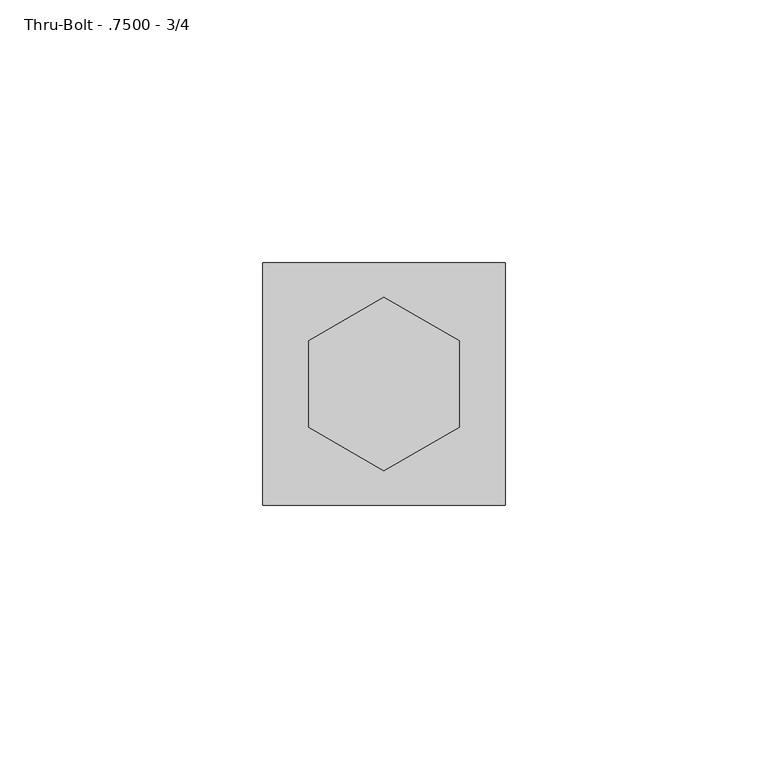
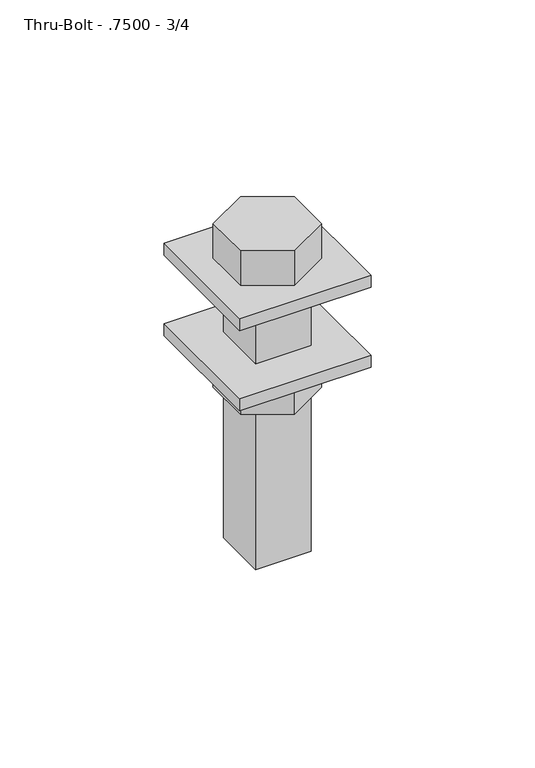
"""IFC4 building model written with IfcOpenShell, lengths in millimetres: fastener geometry, 060523 - W_P_C - Fastenings - Generic - SQUARE : Thru-Bolt - .7500 - 3/4."""

from ifc_helpers import new_model, si_unit, frame, origin, origin_with_axes, place, context, project, spatial, polyline, outline, extrude, source, transform, mapped, element, save


def thru_bolt_7500_3_4_9f574682(model_context):
    return source(origin(), model_context, "Body", "SweptSolid", [
        extrude(outline(polyline([(-23.0683594, -23.0683594), (-23.0683594, 23.0683594), (23.0683594, 23.0683594), (23.0683594, -23.0683594), (-23.0683594, -23.0683594)])), origin_with_axes(), (0.0, 0.0, 1.0), 4.4317708),
        extrude(outline(polyline([(-23.0683594, -23.0683594), (-23.0683594, 23.0683594), (23.0683594, 23.0683594), (23.0683594, -23.0683594), (-23.0683594, -23.0683594)])), frame((0.0, 0.0, -29.8317708), z_axis=(0.0, 0.0, 1.0), x_axis=(1.0, 0.0, 0.0)), (0.0, 0.0, 1.0), 4.4317708),
        extrude(outline(polyline([(-14.2875, -8.248892), (-14.2875, 8.248892), (0.0, 16.4977839), (14.2875, 8.248892), (14.2875, -8.248892), (0.0, -16.4977839), (-14.2875, -8.248892)])), frame((0.0, 0.0, -43.1270833), z_axis=(0.0, 0.0, 1.0), x_axis=(1.0, 0.0, 0.0)), (0.0, 0.0, 1.0), 13.2953125),
        extrude(outline(polyline([(-14.2875, 8.248892), (0.0, 16.4977839), (14.2875, 8.248892), (14.2875, -8.248892), (0.0, -16.4977839), (-14.2875, -8.248892), (-14.2875, 8.248892)])), frame((0.0, 0.0, 4.4317708), z_axis=(0.0, 0.0, 1.0), x_axis=(1.0, 0.0, 0.0)), (0.0, 0.0, 1.0), 13.2953125),
        extrude(outline(polyline([(-9.7730469, 9.7730469), (9.7730469, 9.7730469), (9.7730469, -9.7730469), (-9.7730469, -9.7730469), (-9.7730469, 9.7730469)])), frame((0.0, 0.0, -101.6), z_axis=(0.0, 0.0, 1.0), x_axis=(1.0, 0.0, 0.0)), (0.0, 0.0, 1.0), 106.0317708),
    ])


if __name__ == "__main__":
    model = new_model("IFC4")
    model_context = context("Model", 3, world=origin())
    ifc_project = project(units=[si_unit("LENGTHUNIT", "METRE", prefix="MILLI")], contexts=[model_context])
    site = spatial("IfcSite", under=ifc_project)
    building = spatial("IfcBuilding", under=site)
    placement = place(None, origin())
    thru_bolt_7500_3_4_shape = thru_bolt_7500_3_4_9f574682(model_context)
    element("IfcFastener", 1, ObjectType="060523 - W_P_C - Fastenings - Generic - SQUARE : Thru-Bolt - .7500 - 3/4", at=placement, inside=building, context=model_context, shape_type="MappedRepresentation", body=[
        mapped(thru_bolt_7500_3_4_shape, transform((0.0, 0.0, 0.0), x_axis=(1.0, 0.0, 0.0), y_axis=(0.0, 1.0, 0.0), z_axis=(0.0, 0.0, 1.0))),
    ])
    save(model, "model.ifc")

# Revit data of these elements
# Type "060523 - W_P_C - Fastenings - Generic - SQUARE : Thru-Bolt - .7500 - 3/4"
#   Washer_Thickness = 0' - 0.17448"
#   Washer Radius = 0' - 0.9082"
#   Washer Offset - Head = 0' - 0.17448"
#   Washer Offset = 0' - 0.17448"
#   Thickness_of_Substrate [instance default] = 0' - 1"
#   Side = 0' - 0.65039"
#   Radius = 0' - 0.38477"
#   Length [instance default] = 0' - 4"
#   Head Size = 0' - 1 1/8"
#   Head Radius = 0' - 0 9/16"
#   Head Height = 0' - 0 67/128"
#   Double Diameter = 0' - 1 69/128"
#   Diameter = 0' - 0 197/256"
#   Default Elevation = 4' - 0"
#   Washer_Nut_Visibility = yes
#   Washer_Head_Visibility = yes
#   Round_Head_Visibility = no
#   Point Visibility = no
#   Nut_Visibility = yes
#   Hex_Head_Visiblilty = yes
#   Washer Material = none
#   Bolt Material (Size) = AT SILL - FASTENER AT 24" O.C.
# Element 1 (IfcFastener, "060523 - W_P_C - Fastenings - Generic - SQUARE : Thru-Bolt - .7500 - 3/4")
#   Materials on its faces: "AT SILL - FASTENER AT 24\" O.C."
# Materials
#   "AT SILL - FASTENER AT 24\" O.C.": class "Generic", colour RGB 120 120 120, transparency 0, Cost = 0
